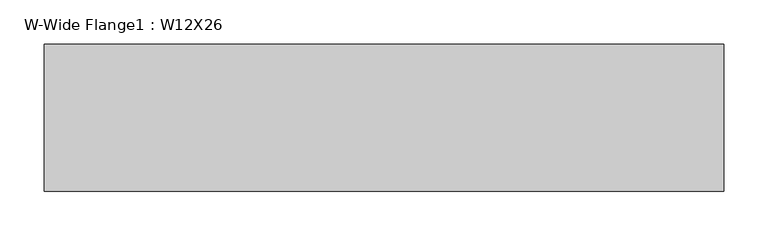
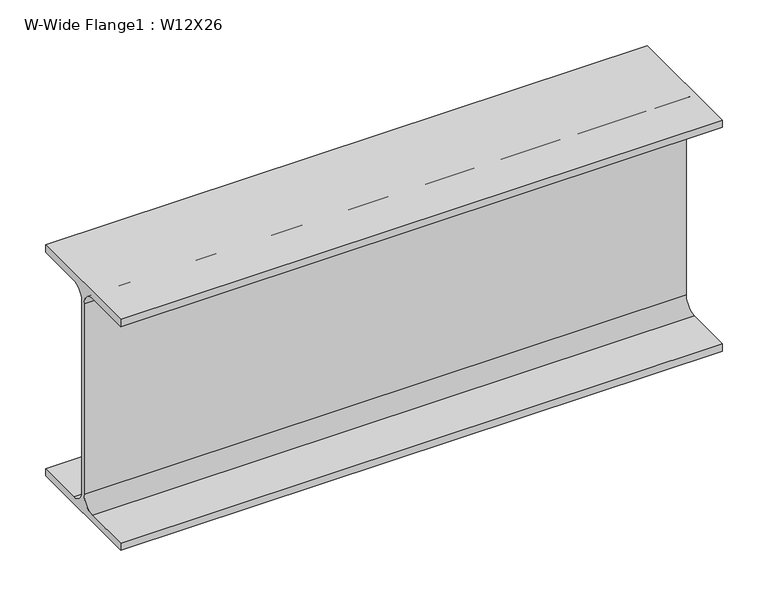
"""IFC4 building model written with IfcOpenShell, lengths in millimetres: beam geometry, W-Wide Flange1 : W12X26."""

from ifc_helpers import new_model, si_unit, point, frame, frame_2d, origin, place, context, project, spatial, polyline, circle_curve, trimmed, segment, composite_curve, outline, extrude, source, transform, mapped, element, save


def w_wide_flange1_w12x26_bb7388ea(model_context):
    return source(origin(), model_context, "Body", "SweptSolid", [
        extrude(outline(composite_curve([segment(polyline([(82.423, -145.288), (82.423, -154.94), (-82.423, -154.94), (-82.423, -145.288), (-20.2565, -145.288)]), True, "CONTINUOUS"), segment(trimmed(circle_curve(frame_2d((-20.2565, -127.9525)), 17.3355), [point((-20.2565, -145.288))], [point((-2.921, -127.9525))], True, "CARTESIAN"), True, "CONTINUOUS"), segment(polyline([(-2.921, -127.9525), (-2.921, 127.9525)]), True, "CONTINUOUS"), segment(trimmed(circle_curve(frame_2d((-20.2565, 127.9525)), 17.3355), [point((-2.921, 127.9525))], [point((-20.2565, 145.288))], True, "CARTESIAN"), True, "CONTINUOUS"), segment(polyline([(-20.2565, 145.288), (-82.423, 145.288), (-82.423, 154.94), (82.423, 154.94), (82.423, 145.288), (20.2565, 145.288)]), True, "CONTINUOUS"), segment(trimmed(circle_curve(frame_2d((20.2565, 127.9525)), 17.3355), [point((20.2565, 145.288))], [point((2.921, 127.9525))], True, "CARTESIAN"), True, "CONTINUOUS"), segment(polyline([(2.921, 127.9525), (2.921, -127.9525)]), True, "CONTINUOUS"), segment(trimmed(circle_curve(frame_2d((20.2565, -127.9525)), 17.3355), [point((2.921, -127.9525))], [point((20.2565, -145.288))], True, "CARTESIAN"), True, "CONTINUOUS"), segment(polyline([(20.2565, -145.288), (82.423, -145.288)]), True, "CONTINUOUS")], self_intersect=False)), frame((-360.1498938, 0.0, 0.0), z_axis=(1.0, 0.0, 0.0), x_axis=(0.0, 1.0, 0.0)), (0.0, 0.0, 1.0), 763.7432001),
    ])


if __name__ == "__main__":
    model = new_model("IFC4")
    model_context = context("Model", 3, world=origin())
    ifc_project = project(units=[si_unit("LENGTHUNIT", "METRE", prefix="MILLI")], contexts=[model_context])
    site = spatial("IfcSite", under=ifc_project)
    building = spatial("IfcBuilding", under=site)
    placement = place(None, origin())
    w_wide_flange1_w12x26_shape = w_wide_flange1_w12x26_bb7388ea(model_context)
    element("IfcBeam", 1, ObjectType="W-Wide Flange1 : W12X26", at=placement, inside=building, context=model_context, shape_type="MappedRepresentation", body=[
        mapped(w_wide_flange1_w12x26_shape, transform((0.0, 0.0, 0.0), x_axis=(1.0, 0.0, 0.0), y_axis=(0.0, 1.0, 0.0), z_axis=(0.0, 0.0, 1.0))),
    ])
    save(model, "model.ifc")

# Revit data of these elements
# Type "W-Wide Flange1 : W12X26"
#   Assembly Code = "B10"
#   W = 26
#   Start Extension Calculation [instance default] = 10' - 0"
#   Start Extension [instance default] = -0' - 0 1/2"
#   End Extension Calculation [instance default] = 10' - 0"
#   End Extension [instance default] = -0' - 0 1/2"
#   Length [instance default] = 5' - 0"
#   bf = 0' - 6.49"
#   d = 1' - 0.2"
#   k = 0' - 1 1/16"
#   k2 = 0' - 0.6825"
#   tf = 0' - 0.38"
#   tw = 0' - 0.23"
#   A = 0.053125 SF
#   Structural Material [instance default] = Metal - Steel - ASTM A992
# Element 1 (IfcBeam, "W-Wide Flange1 : W12X26")
#   Materials on its faces: "Metal - Steel - ASTM A992"
# Materials
#   "Metal - Steel - ASTM A992": class "Metal", colour RGB 199 199 199, transparency 0
